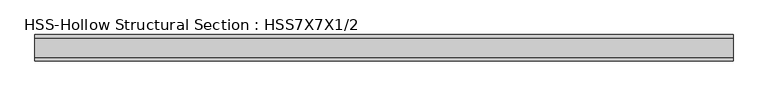
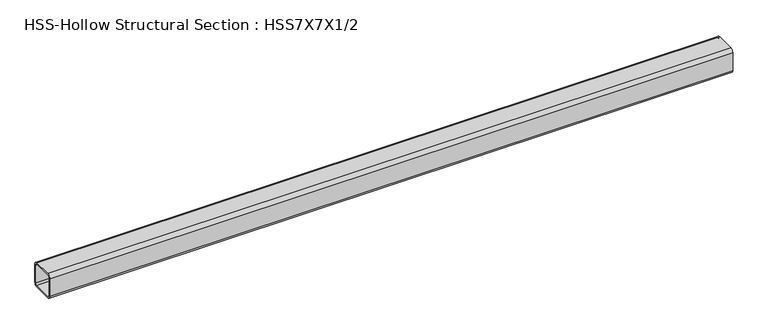
"""IFC4 building model written with IfcOpenShell, lengths in millimetres: member geometry, HSS-Hollow Structural Section : HSS7X7X1/2."""

import ifcopenshell
import ifcopenshell.guid

model = None  # the IFC model being written
_history = None  # IfcOwnerHistory: only IFC2X3 demands one
_inside = {}  # id of a spatial element -> (the spatial element, [elements in it])
_under = {}  # id of a project, library or spatial element -> (it, [spatial elements below it])
_declared = {}  # id of a project -> (the project, [libraries it declares])
_typed = {}  # id of a type object -> (the type object, [elements of that type])
_made_of = {}  # id of a material, layer set ... -> (it, [elements and type objects made of it])


def new_model(schema):
    """Start an empty IFC model of exactly this schema.

    Asked for "IFC4X3", IfcOpenShell would pick the latest addendum, in which some entities
    have other attributes; the version numbers below select the first issue.
    IFC2X3 requires an IfcOwnerHistory on every rooted entity: one is made here for all.
    """
    global model, _history
    if schema == "IFC4X3":
        model = ifcopenshell.file(schema_version=(4, 3, 0, 0))
    else:
        model = ifcopenshell.file(schema=schema)
    _inside.clear()
    _under.clear()
    _declared.clear()
    _typed.clear()
    _made_of.clear()
    _history = None
    if model.schema == "IFC2X3":
        org = make("IfcOrganization", Name="unknown")
        user = make(
            "IfcPersonAndOrganization",
            ThePerson=make("IfcPerson", FamilyName="unknown"),
            TheOrganization=org,
        )
        app = make(
            "IfcApplication",
            ApplicationDeveloper=org,
            Version="unknown",
            ApplicationFullName="unknown",
            ApplicationIdentifier="unknown",
        )
        _history = make(
            "IfcOwnerHistory",
            OwningUser=user,
            OwningApplication=app,
            ChangeAction="ADDED",
            CreationDate=0,
        )
    return model


def make(cls, **values):
    """One entity of the class cls with the attributes given. An attribute that is None is left unset."""
    return model.create_entity(
        cls, **{name: value for name, value in values.items() if value is not None}
    )


def rooted(cls, **values):
    """An entity with a GlobalId (a new one), such as an element, a storey or a relation."""
    return make(cls, GlobalId=ifcopenshell.guid.new(), OwnerHistory=_history, **values)


def si_unit(unit_type, name, prefix=None):
    """IfcSIUnit, for example si_unit("LENGTHUNIT", "METRE", prefix="MILLI")."""
    return make("IfcSIUnit", UnitType=unit_type, Prefix=prefix, Name=name)


def assignment(units):
    """IfcUnitAssignment: the units of a project."""
    return None if units is None else make("IfcUnitAssignment", Units=units)


def point(xyz):
    """IfcCartesianPoint."""
    return None if xyz is None else make("IfcCartesianPoint", Coordinates=xyz)


def direction(xyz):
    """IfcDirection."""
    return None if xyz is None else make("IfcDirection", DirectionRatios=xyz)


def frame(location, z_axis=None, x_axis=None):
    """IfcAxis2Placement3D, a coordinate frame: its origin and axes. An axis left out is left unset."""
    return make(
        "IfcAxis2Placement3D",
        Location=point(location),
        Axis=direction(z_axis),
        RefDirection=direction(x_axis),
    )


def frame_2d(location, x_axis=None):
    """IfcAxis2Placement2D, a coordinate frame in the plane: its origin and x axis."""
    return make(
        "IfcAxis2Placement2D", Location=point(location), RefDirection=direction(x_axis)
    )


def origin():
    """The frame at (0, 0, 0) with its axes left unset."""
    return frame((0.0, 0.0, 0.0))


def place(relative_to, where):
    """IfcLocalPlacement: puts the frame where relative to a parent placement (None: the world)."""
    return make(
        "IfcLocalPlacement", PlacementRelTo=relative_to, RelativePlacement=where
    )


def context(
    kind, dimensions, precision=None, world=None, true_north=None, identifier=None
):
    """IfcGeometricRepresentationContext, for example the 3D "Model" context."""
    return make(
        "IfcGeometricRepresentationContext",
        ContextIdentifier=identifier,
        ContextType=kind,
        CoordinateSpaceDimension=dimensions,
        Precision=precision,
        WorldCoordinateSystem=world,
        TrueNorth=true_north,
    )


def project(units=None, contexts=None):
    """IfcProject with its units and contexts."""
    return rooted(
        "IfcProject",
        Name="project",
        RepresentationContexts=contexts,
        UnitsInContext=assignment(units),
    )


def spatial(cls, under=None, at=None, **own):
    """A site, building, storey or space (cls), placed at a placement, below another one or the project."""
    s = rooted(cls, ObjectPlacement=at, **own)
    if under is not None:
        _under.setdefault(under.id(), (under, []))[1].append(s)
    return s


def polyline(points):
    """IfcPolyline through the points."""
    return make("IfcPolyline", Points=[point(p) for p in points])


def circle_curve(where, radius):
    """IfcCircle in the frame where."""
    return make("IfcCircle", Position=where, Radius=radius)


def trimmed(basis, trim1, trim2, sense, master):
    """IfcTrimmedCurve: the piece of a basis curve between two trims."""
    return make(
        "IfcTrimmedCurve",
        BasisCurve=basis,
        Trim1=trim1,
        Trim2=trim2,
        SenseAgreement=sense,
        MasterRepresentation=master,
    )


def segment(curve, same_sense, transition):
    """IfcCompositeCurveSegment."""
    return make(
        "IfcCompositeCurveSegment",
        Transition=transition,
        SameSense=same_sense,
        ParentCurve=curve,
    )


def composite_curve(segments, self_intersect=None):
    """IfcCompositeCurve: segments joined end to end."""
    return make("IfcCompositeCurve", Segments=segments, SelfIntersect=self_intersect)


def outline(outer, holes=None, kind="AREA"):
    """IfcArbitraryClosedProfileDef: a profile drawn as a closed curve; with holes, ...WithVoids."""
    if holes is None:
        return make("IfcArbitraryClosedProfileDef", ProfileType=kind, OuterCurve=outer)
    return make(
        "IfcArbitraryProfileDefWithVoids",
        ProfileType=kind,
        OuterCurve=outer,
        InnerCurves=holes,
    )


def extrude(swept, where, along, depth):
    """IfcExtrudedAreaSolid: the profile swept, set in the frame where, extruded along a direction by depth."""
    return make(
        "IfcExtrudedAreaSolid",
        SweptArea=swept,
        Position=where,
        ExtrudedDirection=direction(along),
        Depth=depth,
    )


def shape(context_of_items, identifier, shape_type, items):
    """IfcShapeRepresentation: the items that make up one representation, for example the "Body"."""
    return make(
        "IfcShapeRepresentation",
        ContextOfItems=context_of_items,
        RepresentationIdentifier=identifier,
        RepresentationType=shape_type,
        Items=items,
    )


def source(mapping_origin, context_of_items, identifier, shape_type, items):
    """IfcRepresentationMap: a shape defined once, which mapped items show again and again."""
    return make(
        "IfcRepresentationMap",
        MappingOrigin=mapping_origin,
        MappedRepresentation=shape(context_of_items, identifier, shape_type, items),
    )


def transform(
    local_origin,
    x_axis=None,
    y_axis=None,
    z_axis=None,
    scale=None,
    scale2=None,
    scale3=None,
    uniform=True,
):
    """IfcCartesianTransformationOperator3D, or its non-uniform kind. x_axis, y_axis, z_axis: its Axis1, 2, 3."""
    if uniform:
        return make(
            "IfcCartesianTransformationOperator3D",
            Axis1=direction(x_axis),
            Axis2=direction(y_axis),
            LocalOrigin=point(local_origin),
            Scale=scale,
            Axis3=direction(z_axis),
        )
    return make(
        "IfcCartesianTransformationOperator3DnonUniform",
        Axis1=direction(x_axis),
        Axis2=direction(y_axis),
        LocalOrigin=point(local_origin),
        Scale=scale,
        Axis3=direction(z_axis),
        Scale2=scale2,
        Scale3=scale3,
    )


def mapped(mapping_source, mapping_target):
    """IfcMappedItem: shows the shape of a source again, moved by a transform."""
    return make(
        "IfcMappedItem", MappingSource=mapping_source, MappingTarget=mapping_target
    )


def made_of(thing, what):
    """Note that an element or type object is made of a material, layer set ...; save() writes the relation."""
    if what is not None:
        _made_of.setdefault(what.id(), (what, []))[1].append(thing)
    return thing


def element(
    cls,
    number,
    at=None,
    inside=None,
    cuts=None,
    type_object=None,
    material=None,
    context=None,
    identifier="Body",
    shape_type=None,
    held_by="IfcProductDefinitionShape",
    body=None,
    shapes=None,
    **own,
):
    """One element of the class cls, such as IfcWall. Its Tag is "e" and its number.

    at: its placement. inside: the storey or other place that contains it. cuts: it is an
    opening in that element (IfcRelVoidsElement). A single representation is given by context,
    identifier, shape_type and body (its items); several are given by shapes. held_by: the class
    of the entity that holds the representations. save() writes the other relations.
    """
    e = rooted(cls, Tag="e%d" % number, ObjectPlacement=at, **own)
    if body is not None:
        shapes = [shape(context, identifier, shape_type, body)]
    if shapes is not None:
        e.Representation = make(held_by, Representations=shapes)
    if inside is not None:
        _inside.setdefault(inside.id(), (inside, []))[1].append(e)
    if cuts is not None:
        rooted(
            "IfcRelVoidsElement", RelatingBuildingElement=cuts, RelatedOpeningElement=e
        )
    if type_object is not None:
        _typed.setdefault(type_object.id(), (type_object, []))[1].append(e)
    return made_of(e, material)


def aggregate(whole, parts):
    """IfcRelAggregates: a whole, such as a stair, and the parts it consists of."""
    return rooted("IfcRelAggregates", RelatingObject=whole, RelatedObjects=parts)


def save(model, path):
    """Write the relations noted so far, then the file.

    IfcRelAggregates (storeys below a building ...), IfcRelContainedInSpatialStructure (elements
    in a storey), IfcRelDefinesByType, IfcRelAssociatesMaterial and IfcRelDeclares: one each for
    every whole, place, type object, material and project.
    """
    for whole, parts in _under.values():
        aggregate(whole, parts)
    for where, things in _inside.values():
        rooted(
            "IfcRelContainedInSpatialStructure",
            RelatedElements=things,
            RelatingStructure=where,
        )
    for kind, things in _typed.values():
        rooted("IfcRelDefinesByType", RelatedObjects=things, RelatingType=kind)
    for what, things in _made_of.values():
        rooted("IfcRelAssociatesMaterial", RelatedObjects=things, RelatingMaterial=what)
    for by, libraries in _declared.values():
        rooted("IfcRelDeclares", RelatingContext=by, RelatedDefinitions=libraries)
    model.write(path)


def hss_hollow_structural_section_hss7x7x1_2_daed7586(model_context):
    return source(origin(), model_context, "Body", "SweptSolid", [
        extrude(outline(composite_curve([segment(polyline([(88.9, 65.278), (88.9, -65.278)]), True, "CONTINUOUS"), segment(trimmed(circle_curve(frame_2d((65.278, -65.278)), 23.622), [point((88.9, -65.278))], [point((65.278, -88.9))], False, "CARTESIAN"), True, "CONTINUOUS"), segment(polyline([(65.278, -88.9), (-65.278, -88.9)]), True, "CONTINUOUS"), segment(trimmed(circle_curve(frame_2d((-65.278, -65.278)), 23.622), [point((-65.278, -88.9))], [point((-88.9, -65.278))], False, "CARTESIAN"), True, "CONTINUOUS"), segment(polyline([(-88.9, -65.278), (-88.9, 65.278)]), True, "CONTINUOUS"), segment(trimmed(circle_curve(frame_2d((-65.278, 65.278)), 23.622), [point((-88.9, 65.278))], [point((-65.278, 88.9))], False, "CARTESIAN"), True, "CONTINUOUS"), segment(polyline([(-65.278, 88.9), (65.278, 88.9)]), True, "CONTINUOUS"), segment(trimmed(circle_curve(frame_2d((65.278, 65.278)), 23.622), [point((65.278, 88.9))], [point((88.9, 65.278))], False, "CARTESIAN"), True, "CONTINUOUS")], self_intersect=False), holes=[composite_curve([segment(trimmed(circle_curve(frame_2d((-65.278, 65.278)), 11.811), [point((-65.278, 77.089))], [point((-77.089, 65.278))], True, "CARTESIAN"), True, "CONTINUOUS"), segment(polyline([(-77.089, 65.278), (-77.089, -65.278)]), True, "CONTINUOUS"), segment(trimmed(circle_curve(frame_2d((-65.278, -65.278)), 11.811), [point((-77.089, -65.278))], [point((-65.278, -77.089))], True, "CARTESIAN"), True, "CONTINUOUS"), segment(polyline([(-65.278, -77.089), (65.278, -77.089)]), True, "CONTINUOUS"), segment(trimmed(circle_curve(frame_2d((65.278, -65.278)), 11.811), [point((65.278, -77.089))], [point((77.089, -65.278))], True, "CARTESIAN"), True, "CONTINUOUS"), segment(polyline([(77.089, -65.278), (77.089, 65.278)]), True, "CONTINUOUS"), segment(trimmed(circle_curve(frame_2d((65.278, 65.278)), 11.811), [point((77.089, 65.278))], [point((65.278, 77.089))], True, "CARTESIAN"), True, "CONTINUOUS"), segment(polyline([(65.278, 77.089), (-65.278, 77.089)]), True, "CONTINUOUS")], self_intersect=False)]), frame((-2583.6098476, 0.0, 0.0), z_axis=(1.0, 0.0, 0.0), x_axis=(0.0, 1.0, 0.0)), (0.0, 0.0, 1.0), 4736.9581081),
    ])


if __name__ == "__main__":
    model = new_model("IFC4")
    model_context = context("Model", 3, world=origin())
    ifc_project = project(units=[si_unit("LENGTHUNIT", "METRE", prefix="MILLI")], contexts=[model_context])
    site = spatial("IfcSite", under=ifc_project)
    building = spatial("IfcBuilding", under=site)
    placement = place(None, origin())
    hss_hollow_structural_section_hss7x7x1_2_shape = hss_hollow_structural_section_hss7x7x1_2_daed7586(model_context)
    element("IfcMember", 1, ObjectType="HSS-Hollow Structural Section : HSS7X7X1/2", at=placement, inside=building, context=model_context, shape_type="MappedRepresentation", body=[
        mapped(hss_hollow_structural_section_hss7x7x1_2_shape, transform((0.0, 0.0, 0.0), x_axis=(1.0, 0.0, 0.0), y_axis=(0.0, 1.0, 0.0), z_axis=(0.0, 0.0, 1.0))),
    ])
    save(model, "model.ifc")

# Revit data of these elements
# Type "HSS-Hollow Structural Section : HSS7X7X1/2"
#   Assembly Code = "B10"
#   Shape = "Square"
#   W = 41.9
#   Ht = 0' - 7"
#   Length [instance default] = 5' - 0"
#   b = 0' - 7"
#   kr = 0' - 0.93"
#   t = 0' - 0.465"
#   A = 0.0805556 SF
#   Structural Material [instance default] = Steel ASTM A500, Grade B, Rectangular and Square
# Element 1 (IfcMember, "HSS-Hollow Structural Section : HSS7X7X1/2")
#   Materials on its faces: "Steel ASTM A500, Grade B, Rectangular and Square"
# Materials
#   "Steel ASTM A500, Grade B, Rectangular and Square": class "Metal", colour RGB 199 199 199, transparency 0, Description = "Carbon steel", Cost = 0
